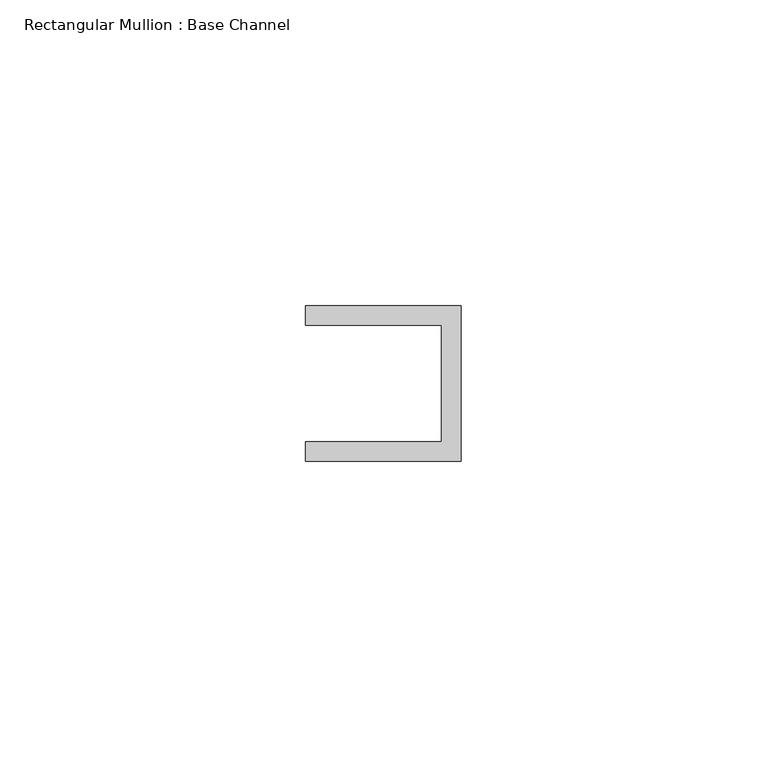
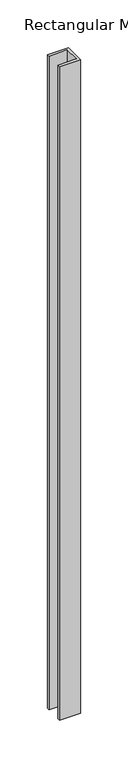
"""IFC4 building model written with IfcOpenShell, lengths in millimetres: member geometry, Rectangular Mullion : Base Channel."""

from ifc_helpers import new_model, si_unit, frame, origin, place, context, project, spatial, polyline, outline, extrude, source, transform, mapped, element, save


def rectangular_mullion_base_channel_13c842bd(model_context):
    return source(origin(), model_context, "Body", "SweptSolid", [
        extrude(outline(polyline([(0.0, -12.7), (-25.4, -12.7), (-25.4, -9.525), (-3.175, -9.525), (-3.175, 9.525), (-25.4, 9.525), (-25.4, 12.7), (0.0, 12.7), (0.0, -12.7)])), frame((0.0, 0.0, -838.1999999), z_axis=(0.0, 0.0, 1.0), x_axis=(1.0, 0.0, 0.0)), (0.0, 0.0, 1.0), 838.1999999),
    ])


if __name__ == "__main__":
    model = new_model("IFC4")
    model_context = context("Model", 3, world=origin())
    ifc_project = project(units=[si_unit("LENGTHUNIT", "METRE", prefix="MILLI")], contexts=[model_context])
    site = spatial("IfcSite", under=ifc_project)
    building = spatial("IfcBuilding", under=site)
    placement = place(None, origin())
    rectangular_mullion_base_channel_shape = rectangular_mullion_base_channel_13c842bd(model_context)
    element("IfcMember", 1, ObjectType="Rectangular Mullion : Base Channel", at=placement, inside=building, context=model_context, shape_type="MappedRepresentation", body=[
        mapped(rectangular_mullion_base_channel_shape, transform((0.0, 0.0, 0.0), x_axis=(1.0, 0.0, 0.0), y_axis=(0.0, 1.0, 0.0), z_axis=(0.0, 0.0, 1.0))),
    ])
    save(model, "model.ifc")

# Revit data of these elements
# Type "Rectangular Mullion : Base Channel"
#   built-in parameter 1007322 = 0.0833333 (stored number, unit not read)
#   built-in parameter 1007321 = 0.0416667 (stored number, unit not read)
#   built-in parameter 1007320 = -0.03125 (stored number, unit not read)
# Element 1 (IfcMember, "Rectangular Mullion : Base Channel")
#   Materials on its faces: "ALUM"
# Materials
#   "ALUM": class "Generic", colour RGB 157 157 157, transparency 0, Cost = 0
